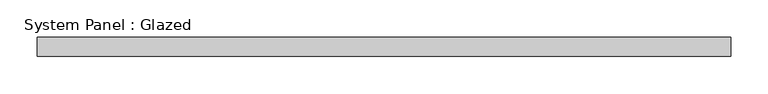
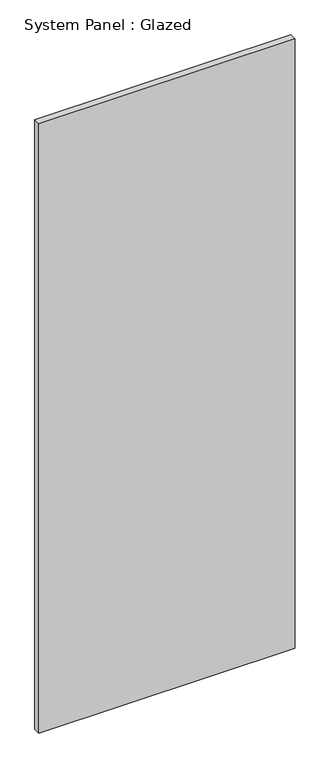
"""IFC4 building model written with IfcOpenShell, lengths in millimetres: plate geometry, System Panel : Glazed."""

from ifc_helpers import new_model, si_unit, origin, origin_with_axes, place, context, project, spatial, polyline, outline, extrude, source, transform, mapped, element, save


def system_panel_glazed_70154507(model_context):
    return source(origin(), model_context, "Body", "SweptSolid", [
        extrude(outline(polyline([(462.5, 24.5), (-462.5, 24.5), (-462.5, 49.5), (462.5, 49.5), (462.5, 24.5)])), origin_with_axes(), (0.0, 0.0, 1.0), 2325.0),
    ])


if __name__ == "__main__":
    model = new_model("IFC4")
    model_context = context("Model", 3, world=origin())
    ifc_project = project(units=[si_unit("LENGTHUNIT", "METRE", prefix="MILLI")], contexts=[model_context])
    site = spatial("IfcSite", under=ifc_project)
    building = spatial("IfcBuilding", under=site)
    placement = place(None, origin())
    system_panel_glazed_shape = system_panel_glazed_70154507(model_context)
    element("IfcPlate", 1, ObjectType="System Panel : Glazed", at=placement, inside=building, context=model_context, shape_type="MappedRepresentation", body=[
        mapped(system_panel_glazed_shape, transform((0.0, 0.0, 0.0), x_axis=(1.0, 0.0, 0.0), y_axis=(0.0, 1.0, 0.0), z_axis=(0.0, 0.0, 1.0))),
    ])
    save(model, "model.ifc")

# Revit data of these elements
# Type "System Panel : Glazed"
#   Construction Type Id = "GSP4R"
#   Analytic Construction = "1/8 in Pilkington single glazing"
#   Visual Light Transmittance = 0.9
#   Solar Heat Gain Coefficient = 0.86
#   Heat Transfer Coefficient (U) = 6.7069 W/(m²·K)
#   Define Thermal Properties by = 1
# Element 1 (IfcPlate, "System Panel : Glazed")
#   Materials on its faces: "Glass"
# Materials
#   "Glass": class "Glass", colour RGB 0 128 192, transparency 0.9, Description = "Soda Lime Glass", Cost = 0
